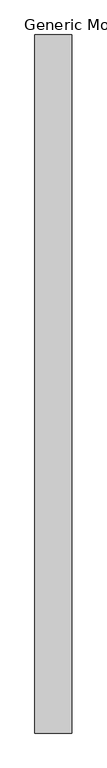
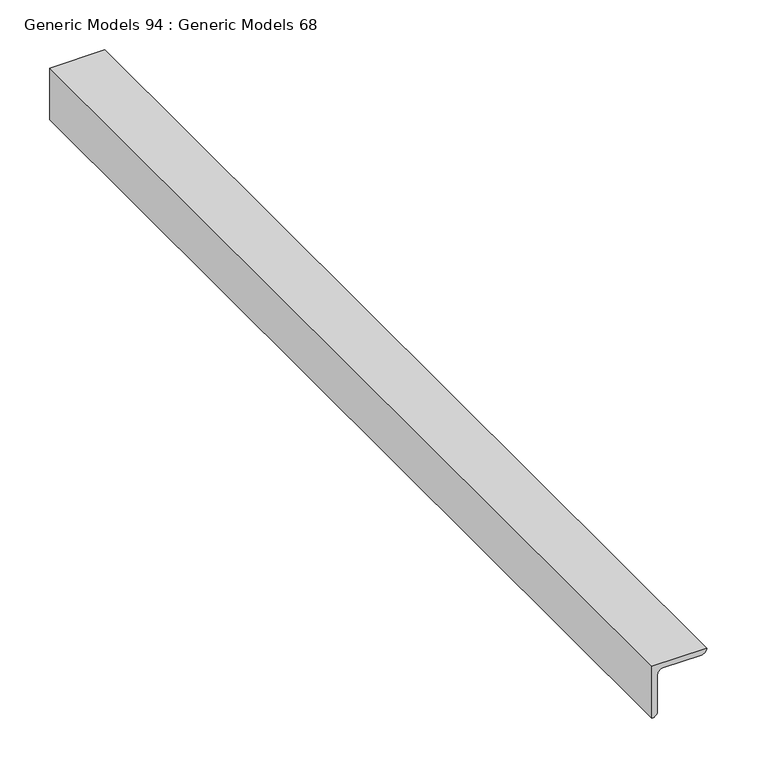
"""IFC4 building model written with IfcOpenShell, lengths in millimetres: proxy geometry, Generic Models 94 : Generic Models 68."""

from ifc_helpers import new_model, si_unit, point, frame, frame_2d, origin, place, context, project, spatial, polyline, circle_curve, trimmed, segment, composite_curve, outline, extrude, source, transform, mapped, element, save


def generic_models_94_generic_models_68_e4309f33(model_context):
    return source(origin(), model_context, "Body", "SweptSolid", [
        extrude(outline(composite_curve([segment(polyline([(266004.6986952, 20536.7616945), (265941.1986952, 20536.7616945)]), True, "CONTINUOUS"), segment(trimmed(circle_curve(frame_2d((265947.5486952, 20536.7616945)), 6.35), [point((265941.1986952, 20536.7616945))], [point((265947.5486952, 20543.1116945))], False, "CARTESIAN"), True, "CONTINUOUS"), segment(polyline([(265947.5486952, 20543.1116945), (265991.9986952, 20543.1116945)]), True, "CONTINUOUS"), segment(trimmed(circle_curve(frame_2d((265991.9986952, 20549.4616945)), 6.35), [point((265991.9986952, 20543.1116945))], [point((265998.3486952, 20549.4616945))], True, "CARTESIAN"), True, "CONTINUOUS"), segment(polyline([(265998.3486952, 20549.4616945), (265998.3486952, 20593.9116945)]), True, "CONTINUOUS"), segment(trimmed(circle_curve(frame_2d((266004.6986952, 20593.9116945)), 6.35), [point((265998.3486952, 20593.9116945))], [point((266004.6986952, 20600.2616945))], False, "CARTESIAN"), True, "CONTINUOUS"), segment(polyline([(266004.6986952, 20600.2616945), (266004.6986952, 20536.7616945)]), True, "CONTINUOUS")], self_intersect=False)), frame((0.0, 17283.1764581, 0.0), z_axis=(0.0, 1.0, 0.0), x_axis=(0.0, 0.0, 1.0)), (0.0, 0.0, 1.0), 1206.5),
    ])


if __name__ == "__main__":
    model = new_model("IFC4")
    model_context = context("Model", 3, world=origin())
    ifc_project = project(units=[si_unit("LENGTHUNIT", "METRE", prefix="MILLI")], contexts=[model_context])
    site = spatial("IfcSite", under=ifc_project)
    building = spatial("IfcBuilding", under=site)
    placement = place(None, origin())
    generic_models_94_generic_models_68_shape = generic_models_94_generic_models_68_e4309f33(model_context)
    element("IfcBuildingElementProxy", 1, Name="Generic Models 94 : Generic Models 68", ObjectType="Generic Models 94 : Generic Models 68", at=placement, inside=building, context=model_context, shape_type="MappedRepresentation", body=[
        mapped(generic_models_94_generic_models_68_shape, transform((0.0, 0.0, 0.0), x_axis=(1.0, 0.0, 0.0), y_axis=(0.0, 1.0, 0.0), z_axis=(0.0, 0.0, 1.0))),
    ])
    save(model, "model.ifc")

# Revit data of these elements
# Element 1 (IfcBuildingElementProxy, "Generic Models 94 : Generic Models 68")
#   Materials on its faces: "CAR DOOR RAIL: GALV. ANGLE L2 1/2 X 2 1/2 X 1/4\" @ 32\" ABOVE GRADE (PARALLEL TO HORTZ. WOOD TRIM)"
# Materials
#   "CAR DOOR RAIL: GALV. ANGLE L2 1/2 X 2 1/2 X 1/4\" @ 32\" ABOVE GRADE (PARALLEL TO HORTZ. WOOD TRIM)": class "Unassigned", colour RGB 211 211 211, transparency 0, Cost = 0
